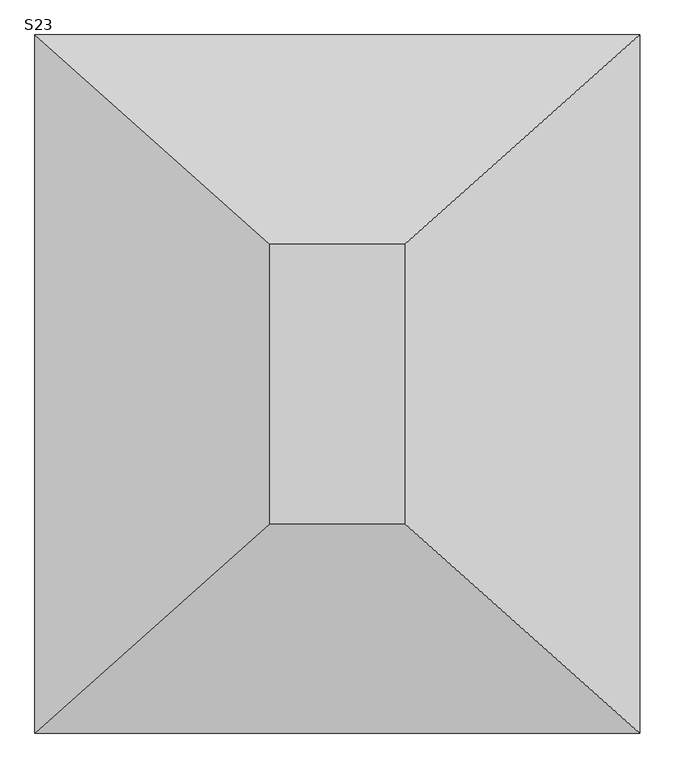
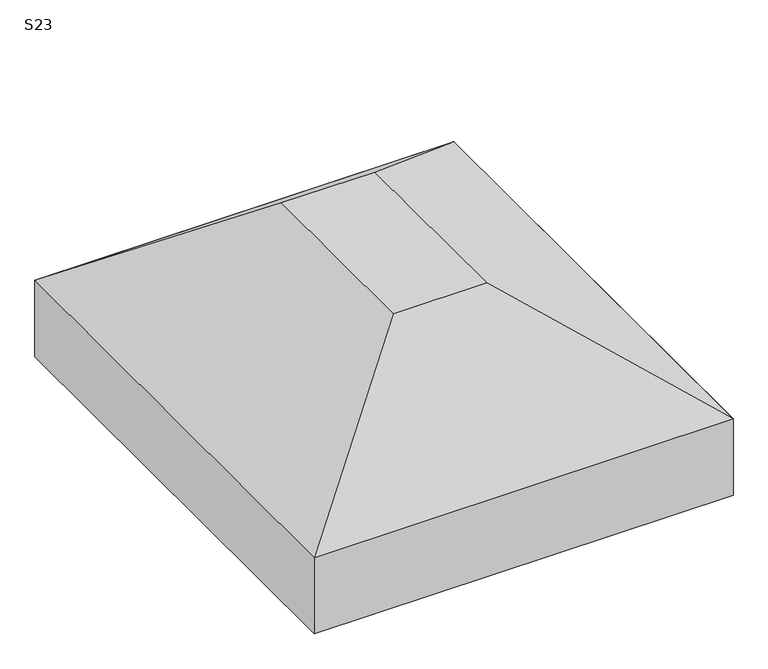
"""IFC4 building model written with IfcOpenShell, lengths in millimetres: fastener geometry, TQS - Sapata : S23."""

from ifc_helpers import new_model, si_unit, frame, origin, place, context, project, spatial, polyline, outline, extrude, faceted_brep, source, transform, mapped, element, save


def s23_c1a85685(model_context):
    return source(origin(), model_context, "Body", "SolidModel", [
        faceted_brep([(-55.0, 100.0, 0.0), (-345.0, 100.0, 0.0), (-345.0, -500.0, 0.0), (-55.0, -500.0, 0.0), (450.0, 550.0, -350.0), (450.0, -950.0, -350.0), (-850.0, -950.0, -350.0), (-850.0, 550.0, -350.0)], [[[0, 1, 2, 3]], [[4, 5, 6, 7]], [[4, 7, 1, 0]], [[7, 6, 2, 1]], [[6, 5, 3, 2]], [[5, 4, 0, 3]]]),
        extrude(outline(polyline([(450.0, 550.0), (450.0, -950.0), (-850.0, -950.0), (-850.0, 550.0), (450.0, 550.0)])), frame((0.0, 0.0, -600.0), z_axis=(0.0, 0.0, 1.0), x_axis=(1.0, 0.0, 0.0)), (0.0, 0.0, 1.0), 250.0),
    ])


if __name__ == "__main__":
    model = new_model("IFC4")
    model_context = context("Model", 3, world=origin())
    ifc_project = project(units=[si_unit("LENGTHUNIT", "METRE", prefix="MILLI")], contexts=[model_context])
    site = spatial("IfcSite", under=ifc_project)
    building = spatial("IfcBuilding", under=site)
    placement = place(None, origin())
    s23_shape = s23_c1a85685(model_context)
    element("IfcFastener", 1, ObjectType="TQS - Sapata : S23", at=placement, inside=building, context=model_context, shape_type="MappedRepresentation", body=[
        mapped(s23_shape, transform((0.0, 0.0, 0.0), x_axis=(1.0, 0.0, 0.0), y_axis=(0.0, 1.0, 0.0), z_axis=(0.0, 0.0, 1.0))),
    ])
    save(model, "model.ifc")

# Revit data of these elements
# Type "TQS - Sapata : S23"
#   TY = 0.60 m
#   TX = 0.29 m
#   HS = 0.60 m
#   H0 = 0.25 m
#   EXCYABS = 0.75 m
#   EXCY = 0.00 m
#   EXCXABS = 0.65 m
#   EXCX = 0.00 m
#   DIMY = 1.50 m
#   DIMX = 1.30 m
#   Material estrutural = Concreto - Concreto concretado no local
#   Width = 0
#   Length = 0
# Element 1 (IfcFastener, "TQS - Sapata : S23")
#   Materials on its faces: "Concreto - Concreto concretado no local"
# Materials
#   "Concreto - Concreto concretado no local": class "Concreto", colour RGB 192 192 192, transparency 0
